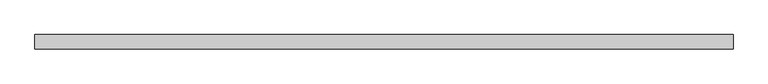
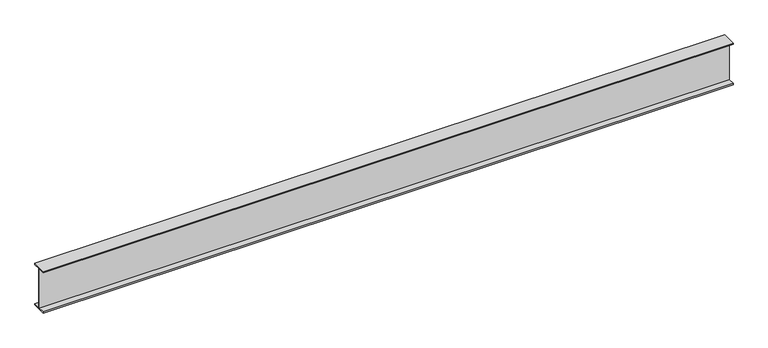
"""IFC4 building model written with IfcOpenShell, lengths in millimetres: proxy geometry, Generic Models 7:Generic Models 1:8:Generic Models 1:8 : Generic Models 7:Generic Models 1:337419:4 : Generic Models 7:Generic Models 1:8:Generic Models 1:8 : Generic Models 7:Generic Models 1:337419:315935."""

from ifc_helpers import new_model, si_unit, frame, origin, place, context, project, spatial, polyline, outline, extrude, source, transform, mapped, element, save


def generic_models_a9831ab9(model_context):
    return source(origin(), model_context, "Body", "SweptSolid", [
        extrude(outline(polyline([(-578721.4183841, 3684.9579167), (-578721.4183841, 3693.8479167), (-578619.5643841, 3693.8479167), (-578619.5643841, 3684.9579167), (-578667.5068841, 3684.9579167), (-578667.5068841, 3392.8579167), (-578619.5643841, 3392.8579167), (-578619.5643841, 3383.9679167), (-578721.4183841, 3383.9679167), (-578721.4183841, 3392.8579167), (-578673.4758841, 3392.8579167), (-578673.4758841, 3684.9579167), (-578721.4183841, 3684.9579167)])), frame((591306.0367239, 0.0, 0.0), z_axis=(1.0, 0.0, 0.0), x_axis=(0.0, 1.0, 0.0)), (0.0, 0.0, 1.0), 4876.8),
    ])


if __name__ == "__main__":
    model = new_model("IFC4")
    model_context = context("Model", 3, world=origin())
    ifc_project = project(units=[si_unit("LENGTHUNIT", "METRE", prefix="MILLI")], contexts=[model_context])
    site = spatial("IfcSite", under=ifc_project)
    building = spatial("IfcBuilding", under=site)
    placement = place(None, origin())
    generic_models_shape = generic_models_a9831ab9(model_context)
    element("IfcBuildingElementProxy", 1, Name="Generic Models 7:Generic Models 1:8:Generic Models 1:8 : Generic Models 7:Generic Models 1:337419:4 : Generic Models 7:Generic Models 1:8:Generic Models 1:8 : Generic Models 7:Generic Models 1:337419:315935", ObjectType="Generic Models 7:Generic Models 1:8:Generic Models 1:8 : Generic Models 7:Generic Models 1:337419:4 : Generic Models 7:Generic Models 1:8:Generic Models 1:8 : Generic Models 7:Generic Models 1:337419:315935", at=placement, inside=building, context=model_context, shape_type="MappedRepresentation", body=[
        mapped(generic_models_shape, transform((0.0, 0.0, 0.0), x_axis=(1.0, 0.0, 0.0), y_axis=(0.0, 1.0, 0.0), z_axis=(0.0, 0.0, 1.0))),
    ])
    save(model, "model.ifc")

# Revit data of these elements
# Type "Generic Models 7:Generic Models 1:8:Generic Models 1:8 : Generic Models 7:Generic Models 1:337419:4 : Generic Models 7:Generic Models 1:8:Generic Models 1:8 : Generic Models 7:Generic Models 1:337419:315935"
#   NameOverride = "Generic Models 7:Generic Models 1:8:Generic Models 1:8 : Generic Models 7:Generic Models 1:337419:315935"
#   ObjectTypeOverride = "Generic Models 1:8 : Generic Models 7:Generic Models 1:337419"
#   Reference = "Generic Models 1"
#   Tag = "315935"
# Element 1 (IfcBuildingElementProxy, "Generic Models 7:Generic Models 1:8:Generic Models 1:8 : Generic Models 7:Generic Models 1:337419:4 : Generic Models 7:Generic Models 1:8:Generic Models 1:8 : Generic Models 7:Generic Models 1:337419:315935")
#   Materials on its faces: "STRUCTURAL STEEL - SEE STRUCT. DWGS"
# Materials
#   "STRUCTURAL STEEL - SEE STRUCT. DWGS": class "Metal", colour RGB 189 187 185, transparency 0, Description = "Structural steel 50ksi", Cost = 0
